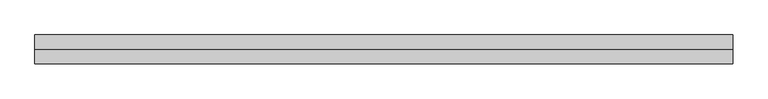
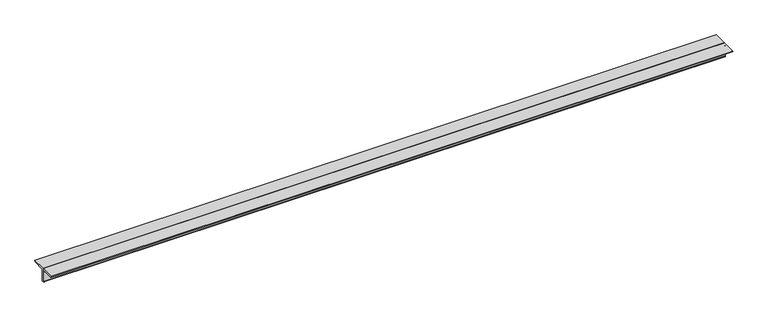
"""IFC4 building model written with IfcOpenShell, lengths in millimetres: member geometry, Steel Framing_2Ls_KS : H_SB_AR_S02_2Ls-100x100x10_VBR1."""

from ifc_helpers import new_model, si_unit, point, frame, frame_2d, origin, place, context, project, spatial, polyline, circle_curve, trimmed, segment, composite_curve, outline, extrude, source, transform, mapped, element, save


def member_c0fb5a4a(model_context):
    return source(origin(), model_context, "Body", "SweptSolid", [
        extrude(outline(composite_curve([segment(polyline([(0.0, 28.2), (100.0, 28.2)]), True, "CONTINUOUS"), segment(trimmed(circle_curve(frame_2d((90.0, 28.2)), 10.0), [point((100.0, 28.2))], [point((90.0, 18.2))], False, "CARTESIAN"), True, "CONTINUOUS"), segment(polyline([(90.0, 18.2), (20.0, 18.2)]), True, "CONTINUOUS"), segment(trimmed(circle_curve(frame_2d((20.0, 8.2)), 10.0), [point((20.0, 18.2))], [point((10.0, 8.2))], True, "CARTESIAN"), True, "CONTINUOUS"), segment(polyline([(10.0, 8.2), (10.0, -61.8)]), True, "CONTINUOUS"), segment(trimmed(circle_curve(frame_2d((0.0, -61.8)), 10.0), [point((10.0, -61.8))], [point((0.0, -71.8))], False, "CARTESIAN"), True, "CONTINUOUS"), segment(polyline([(0.0, -71.8), (0.0, 28.2)]), True, "CONTINUOUS")], self_intersect=False)), frame((-2479.1576866, 0.0, 0.0), z_axis=(1.0, 0.0, 0.0), x_axis=(0.0, 1.0, 0.0)), (0.0, 0.0, 1.0), 4834.643543),
        extrude(outline(composite_curve([segment(polyline([(0.0, 28.2), (0.0, -71.8)]), True, "CONTINUOUS"), segment(trimmed(circle_curve(frame_2d((0.0, -61.8)), 10.0), [point((0.0, -71.8))], [point((-10.0, -61.8))], False, "CARTESIAN"), True, "CONTINUOUS"), segment(polyline([(-10.0, -61.8), (-10.0, 8.2)]), True, "CONTINUOUS"), segment(trimmed(circle_curve(frame_2d((-20.0, 8.2)), 10.0), [point((-10.0, 8.2))], [point((-20.0, 18.2))], True, "CARTESIAN"), True, "CONTINUOUS"), segment(polyline([(-20.0, 18.2), (-90.0, 18.2)]), True, "CONTINUOUS"), segment(trimmed(circle_curve(frame_2d((-90.0, 28.2)), 10.0), [point((-90.0, 18.2))], [point((-100.0, 28.2))], False, "CARTESIAN"), True, "CONTINUOUS"), segment(polyline([(-100.0, 28.2), (0.0, 28.2)]), True, "CONTINUOUS")], self_intersect=False)), frame((-2479.1576866, 0.0, 0.0), z_axis=(1.0, 0.0, 0.0), x_axis=(0.0, 1.0, 0.0)), (0.0, 0.0, 1.0), 4834.643543),
    ])


if __name__ == "__main__":
    model = new_model("IFC4")
    model_context = context("Model", 3, world=origin())
    ifc_project = project(units=[si_unit("LENGTHUNIT", "METRE", prefix="MILLI")], contexts=[model_context])
    site = spatial("IfcSite", under=ifc_project)
    building = spatial("IfcBuilding", under=site)
    placement = place(None, origin())
    member_shape = member_c0fb5a4a(model_context)
    element("IfcMember", 1, ObjectType="Steel Framing_2Ls_KS : H_SB_AR_S02_2Ls-100x100x10_VBR1", at=placement, inside=building, context=model_context, shape_type="MappedRepresentation", body=[
        mapped(member_shape, transform((0.0, 0.0, 0.0), x_axis=(1.0, 0.0, 0.0), y_axis=(0.0, 1.0, 0.0), z_axis=(0.0, 0.0, 1.0))),
    ])
    save(model, "model.ifc")

# Revit data of these elements
# Type "Steel Framing_2Ls_KS : H_SB_AR_S02_2Ls-100x100x10_VBR1"
#   Type Comments = "MAIN"
#   Type Mark = "VBR1"
#   H_SectionID = "2Ls-100x100x10"
#   Assembly Code = "B10"
#   Legs = "LLBB"
#   H_Ratio for Additional Steel Plate = 0.2
#   W = 0
#   Perimeter = 0.80 m²/m
#   Nominal Weight = 29.80 kgf/m
#   Length [instance default] = 1524 mm
#   Space = 0 mm
#   b = 100 mm
#   d = 100 mm
#   t = 10 mm
#   y = 28.2 mm
#   A = 0.0038 m²
#   Structural Material [instance default] = Steel, 45-345
# Element 1 (IfcMember, "Steel Framing_2Ls_KS : H_SB_AR_S02_2Ls-100x100x10_VBR1")
#   Materials on its faces: "Steel, 45-345"
# Materials
#   "Steel, 45-345": class "Metal", colour RGB 189 187 185, transparency 0, Description = "Steel 345 MPa", Cost = 0
